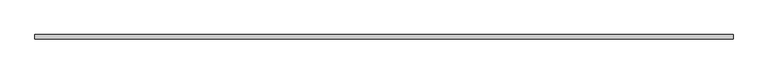
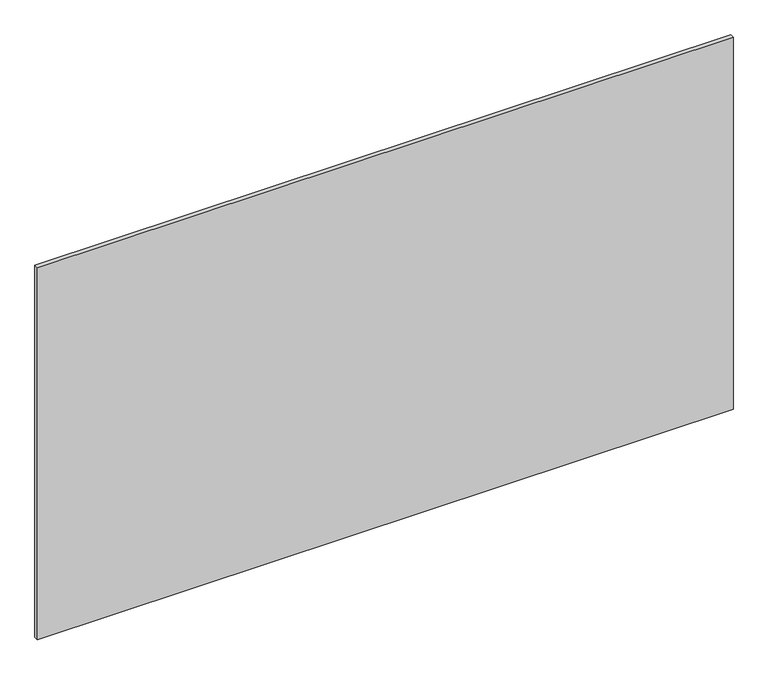
"""IFC4 building model written with IfcOpenShell, lengths in millimetres: railing geometry, ML_Painéis1 : ML_Painéis."""

import ifcopenshell
import ifcopenshell.guid

model = None  # the IFC model being written
_history = None  # IfcOwnerHistory: only IFC2X3 demands one
_inside = {}  # id of a spatial element -> (the spatial element, [elements in it])
_under = {}  # id of a project, library or spatial element -> (it, [spatial elements below it])
_declared = {}  # id of a project -> (the project, [libraries it declares])
_typed = {}  # id of a type object -> (the type object, [elements of that type])
_made_of = {}  # id of a material, layer set ... -> (it, [elements and type objects made of it])


def new_model(schema):
    """Start an empty IFC model of exactly this schema.

    Asked for "IFC4X3", IfcOpenShell would pick the latest addendum, in which some entities
    have other attributes; the version numbers below select the first issue.
    IFC2X3 requires an IfcOwnerHistory on every rooted entity: one is made here for all.
    """
    global model, _history
    if schema == "IFC4X3":
        model = ifcopenshell.file(schema_version=(4, 3, 0, 0))
    else:
        model = ifcopenshell.file(schema=schema)
    _inside.clear()
    _under.clear()
    _declared.clear()
    _typed.clear()
    _made_of.clear()
    _history = None
    if model.schema == "IFC2X3":
        org = make("IfcOrganization", Name="unknown")
        user = make(
            "IfcPersonAndOrganization",
            ThePerson=make("IfcPerson", FamilyName="unknown"),
            TheOrganization=org,
        )
        app = make(
            "IfcApplication",
            ApplicationDeveloper=org,
            Version="unknown",
            ApplicationFullName="unknown",
            ApplicationIdentifier="unknown",
        )
        _history = make(
            "IfcOwnerHistory",
            OwningUser=user,
            OwningApplication=app,
            ChangeAction="ADDED",
            CreationDate=0,
        )
    return model


def make(cls, **values):
    """One entity of the class cls with the attributes given. An attribute that is None is left unset."""
    return model.create_entity(
        cls, **{name: value for name, value in values.items() if value is not None}
    )


def rooted(cls, **values):
    """An entity with a GlobalId (a new one), such as an element, a storey or a relation."""
    return make(cls, GlobalId=ifcopenshell.guid.new(), OwnerHistory=_history, **values)


def si_unit(unit_type, name, prefix=None):
    """IfcSIUnit, for example si_unit("LENGTHUNIT", "METRE", prefix="MILLI")."""
    return make("IfcSIUnit", UnitType=unit_type, Prefix=prefix, Name=name)


def assignment(units):
    """IfcUnitAssignment: the units of a project."""
    return None if units is None else make("IfcUnitAssignment", Units=units)


def point(xyz):
    """IfcCartesianPoint."""
    return None if xyz is None else make("IfcCartesianPoint", Coordinates=xyz)


def direction(xyz):
    """IfcDirection."""
    return None if xyz is None else make("IfcDirection", DirectionRatios=xyz)


def frame(location, z_axis=None, x_axis=None):
    """IfcAxis2Placement3D, a coordinate frame: its origin and axes. An axis left out is left unset."""
    return make(
        "IfcAxis2Placement3D",
        Location=point(location),
        Axis=direction(z_axis),
        RefDirection=direction(x_axis),
    )


def origin():
    """The frame at (0, 0, 0) with its axes left unset."""
    return frame((0.0, 0.0, 0.0))


def place(relative_to, where):
    """IfcLocalPlacement: puts the frame where relative to a parent placement (None: the world)."""
    return make(
        "IfcLocalPlacement", PlacementRelTo=relative_to, RelativePlacement=where
    )


def context(
    kind, dimensions, precision=None, world=None, true_north=None, identifier=None
):
    """IfcGeometricRepresentationContext, for example the 3D "Model" context."""
    return make(
        "IfcGeometricRepresentationContext",
        ContextIdentifier=identifier,
        ContextType=kind,
        CoordinateSpaceDimension=dimensions,
        Precision=precision,
        WorldCoordinateSystem=world,
        TrueNorth=true_north,
    )


def project(units=None, contexts=None):
    """IfcProject with its units and contexts."""
    return rooted(
        "IfcProject",
        Name="project",
        RepresentationContexts=contexts,
        UnitsInContext=assignment(units),
    )


def spatial(cls, under=None, at=None, **own):
    """A site, building, storey or space (cls), placed at a placement, below another one or the project."""
    s = rooted(cls, ObjectPlacement=at, **own)
    if under is not None:
        _under.setdefault(under.id(), (under, []))[1].append(s)
    return s


def polyline(points):
    """IfcPolyline through the points."""
    return make("IfcPolyline", Points=[point(p) for p in points])


def outline(outer, holes=None, kind="AREA"):
    """IfcArbitraryClosedProfileDef: a profile drawn as a closed curve; with holes, ...WithVoids."""
    if holes is None:
        return make("IfcArbitraryClosedProfileDef", ProfileType=kind, OuterCurve=outer)
    return make(
        "IfcArbitraryProfileDefWithVoids",
        ProfileType=kind,
        OuterCurve=outer,
        InnerCurves=holes,
    )


def extrude(swept, where, along, depth):
    """IfcExtrudedAreaSolid: the profile swept, set in the frame where, extruded along a direction by depth."""
    return make(
        "IfcExtrudedAreaSolid",
        SweptArea=swept,
        Position=where,
        ExtrudedDirection=direction(along),
        Depth=depth,
    )


def shape(context_of_items, identifier, shape_type, items):
    """IfcShapeRepresentation: the items that make up one representation, for example the "Body"."""
    return make(
        "IfcShapeRepresentation",
        ContextOfItems=context_of_items,
        RepresentationIdentifier=identifier,
        RepresentationType=shape_type,
        Items=items,
    )


def source(mapping_origin, context_of_items, identifier, shape_type, items):
    """IfcRepresentationMap: a shape defined once, which mapped items show again and again."""
    return make(
        "IfcRepresentationMap",
        MappingOrigin=mapping_origin,
        MappedRepresentation=shape(context_of_items, identifier, shape_type, items),
    )


def transform(
    local_origin,
    x_axis=None,
    y_axis=None,
    z_axis=None,
    scale=None,
    scale2=None,
    scale3=None,
    uniform=True,
):
    """IfcCartesianTransformationOperator3D, or its non-uniform kind. x_axis, y_axis, z_axis: its Axis1, 2, 3."""
    if uniform:
        return make(
            "IfcCartesianTransformationOperator3D",
            Axis1=direction(x_axis),
            Axis2=direction(y_axis),
            LocalOrigin=point(local_origin),
            Scale=scale,
            Axis3=direction(z_axis),
        )
    return make(
        "IfcCartesianTransformationOperator3DnonUniform",
        Axis1=direction(x_axis),
        Axis2=direction(y_axis),
        LocalOrigin=point(local_origin),
        Scale=scale,
        Axis3=direction(z_axis),
        Scale2=scale2,
        Scale3=scale3,
    )


def mapped(mapping_source, mapping_target):
    """IfcMappedItem: shows the shape of a source again, moved by a transform."""
    return make(
        "IfcMappedItem", MappingSource=mapping_source, MappingTarget=mapping_target
    )


def made_of(thing, what):
    """Note that an element or type object is made of a material, layer set ...; save() writes the relation."""
    if what is not None:
        _made_of.setdefault(what.id(), (what, []))[1].append(thing)
    return thing


def element(
    cls,
    number,
    at=None,
    inside=None,
    cuts=None,
    type_object=None,
    material=None,
    context=None,
    identifier="Body",
    shape_type=None,
    held_by="IfcProductDefinitionShape",
    body=None,
    shapes=None,
    **own,
):
    """One element of the class cls, such as IfcWall. Its Tag is "e" and its number.

    at: its placement. inside: the storey or other place that contains it. cuts: it is an
    opening in that element (IfcRelVoidsElement). A single representation is given by context,
    identifier, shape_type and body (its items); several are given by shapes. held_by: the class
    of the entity that holds the representations. save() writes the other relations.
    """
    e = rooted(cls, Tag="e%d" % number, ObjectPlacement=at, **own)
    if body is not None:
        shapes = [shape(context, identifier, shape_type, body)]
    if shapes is not None:
        e.Representation = make(held_by, Representations=shapes)
    if inside is not None:
        _inside.setdefault(inside.id(), (inside, []))[1].append(e)
    if cuts is not None:
        rooted(
            "IfcRelVoidsElement", RelatingBuildingElement=cuts, RelatedOpeningElement=e
        )
    if type_object is not None:
        _typed.setdefault(type_object.id(), (type_object, []))[1].append(e)
    return made_of(e, material)


def aggregate(whole, parts):
    """IfcRelAggregates: a whole, such as a stair, and the parts it consists of."""
    return rooted("IfcRelAggregates", RelatingObject=whole, RelatedObjects=parts)


def save(model, path):
    """Write the relations noted so far, then the file.

    IfcRelAggregates (storeys below a building ...), IfcRelContainedInSpatialStructure (elements
    in a storey), IfcRelDefinesByType, IfcRelAssociatesMaterial and IfcRelDeclares: one each for
    every whole, place, type object, material and project.
    """
    for whole, parts in _under.values():
        aggregate(whole, parts)
    for where, things in _inside.values():
        rooted(
            "IfcRelContainedInSpatialStructure",
            RelatedElements=things,
            RelatingStructure=where,
        )
    for kind, things in _typed.values():
        rooted("IfcRelDefinesByType", RelatedObjects=things, RelatingType=kind)
    for what, things in _made_of.values():
        rooted("IfcRelAssociatesMaterial", RelatedObjects=things, RelatingMaterial=what)
    for by, libraries in _declared.values():
        rooted("IfcRelDeclares", RelatingContext=by, RelatedDefinitions=libraries)
    model.write(path)


def railing_50812a2e(model_context):
    return source(origin(), model_context, "Body", "SweptSolid", [
        extrude(outline(polyline([(-4674.5702584, 2133.3602771), (-4674.5702584, 2121.3602771), (-6620.5702584, 2121.3602771), (-6620.5702584, 2133.3602771), (-4674.5702584, 2133.3602771)])), frame((0.0, 0.0, 4122.0679199), z_axis=(0.0, 0.0, 1.0), x_axis=(1.0, 0.0, 0.0)), (0.0, 0.0, 1.0), 1100.0),
    ])


if __name__ == "__main__":
    model = new_model("IFC4")
    model_context = context("Model", 3, world=origin())
    ifc_project = project(units=[si_unit("LENGTHUNIT", "METRE", prefix="MILLI")], contexts=[model_context])
    site = spatial("IfcSite", under=ifc_project)
    building = spatial("IfcBuilding", under=site)
    placement = place(None, origin())
    railing_shape = railing_50812a2e(model_context)
    element("IfcRailing", 1, ObjectType="ML_Painéis1 : ML_Painéis", at=placement, inside=building, context=model_context, shape_type="MappedRepresentation", body=[
        mapped(railing_shape, transform((0.0, 0.0, 0.0), x_axis=(1.0, 0.0, 0.0), y_axis=(0.0, 1.0, 0.0), z_axis=(0.0, 0.0, 1.0))),
    ])
    save(model, "model.ifc")

# Revit data of these elements
# Type "ML_Painéis1 : ML_Painéis"
#   ME_Área [instance default] = 2.1406 m²
#   ME_Espessura [instance default] = 0.012 m
#   ME_Dist Painéis [instance default] = 0.002 m
#   ME_Compr Painéis [instance default] = 1.946 m
#   ME_Compr [instance default] = 1.95 m
#   ME_Altura [instance default] = 1.10 m
#   ME_Quant Painéis [instance default] = 3
#   ME_Painel Único [instance default] = yes
#   ME_Paineis Vários [instance default] = no
#   ME_Material Tipo Vidro [instance default] = .VIDRO GENÉRICO
# Element 1 (IfcRailing, "ML_Painéis1 : ML_Painéis")
#   Materials on its faces: ".VIDRO GENÉRICO"
# Materials
#   ".VIDRO GENÉRICO": class ".CC_VIDRO", colour RGB 0 128 192, transparency 0.9, Description = "Vidro comum", Cost = 0
